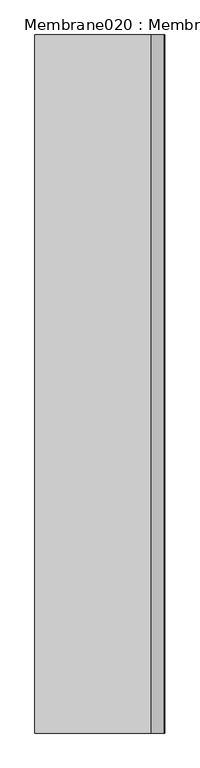
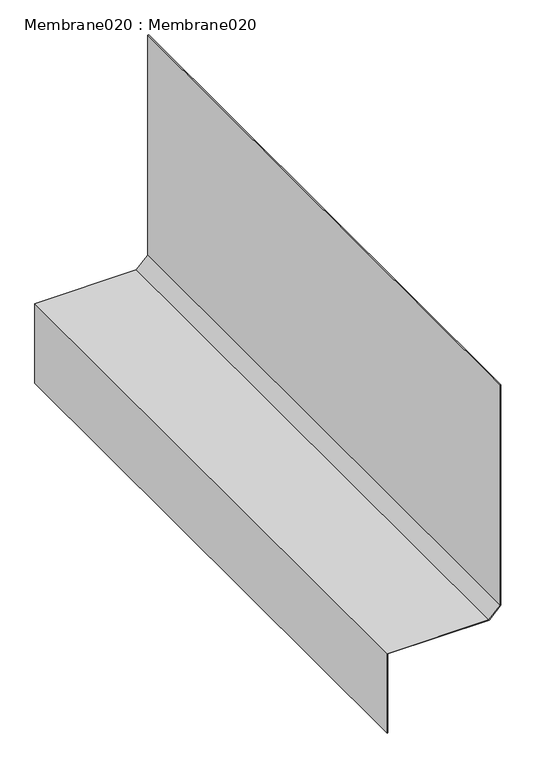
"""IFC4 building model written with IfcOpenShell, lengths in millimetres: proxy geometry, Membrane020 : Membrane020."""

from ifc_helpers import new_model, si_unit, frame, origin, place, context, project, spatial, polyline, outline, extrude, source, transform, mapped, element, save


def membrane020_membrane020_6a48586c(model_context):
    return source(origin(), model_context, "Body", "SweptSolid", [
        extrude(outline(polyline([(33390.8554688, -9667.8427734), (32628.5272919, -9667.8427734), (32590.4931641, -9705.461443), (32590.4931641, -10038.2705078), (32314.8961275, -10038.2705078), (32314.8961275, -10036.2705078), (32588.4931641, -10036.2705078), (32588.4931641, -9704.6265747), (32627.7052912, -9665.8427734), (33390.8554688, -9665.8427734), (33390.8554688, -9667.8427734)])), frame((0.0, 7982.1531721, 0.0), z_axis=(0.0, 1.0, 0.0), x_axis=(0.0, 0.0, 1.0)), (0.0, 0.0, 1.0), 2000.0),
    ])


if __name__ == "__main__":
    model = new_model("IFC4")
    model_context = context("Model", 3, world=origin())
    ifc_project = project(units=[si_unit("LENGTHUNIT", "METRE", prefix="MILLI")], contexts=[model_context])
    site = spatial("IfcSite", under=ifc_project)
    building = spatial("IfcBuilding", under=site)
    placement = place(None, origin())
    membrane020_membrane020_shape = membrane020_membrane020_6a48586c(model_context)
    element("IfcBuildingElementProxy", 1, Name="Membrane020 : Membrane020", ObjectType="Membrane020 : Membrane020", at=placement, inside=building, context=model_context, shape_type="MappedRepresentation", body=[
        mapped(membrane020_membrane020_shape, transform((0.0, 0.0, 0.0), x_axis=(1.0, 0.0, 0.0), y_axis=(0.0, 1.0, 0.0), z_axis=(0.0, 0.0, 1.0))),
    ])
    save(model, "model.ifc")

# Revit data of these elements
# Type "Membrane020 : Membrane020"
#   NameOverride = "Membrane020"
# Element 1 (IfcBuildingElementProxy, "Membrane020 : Membrane020")
#   Materials on its faces: "ECO ROOT BARRIER"
# Materials
#   "ECO ROOT BARRIER": class "Unassigned", colour RGB 135 255 2, transparency 0
